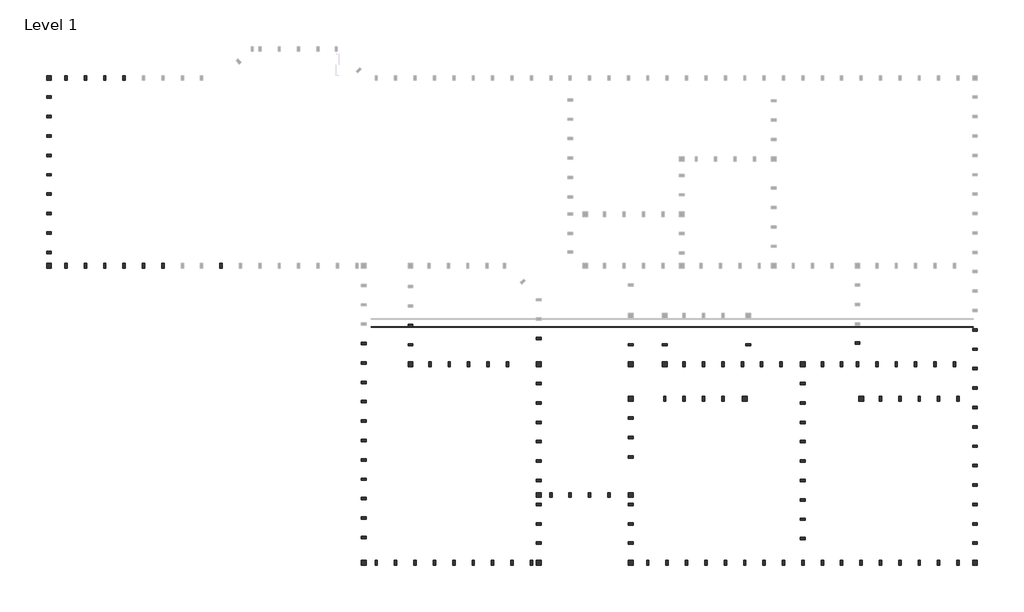
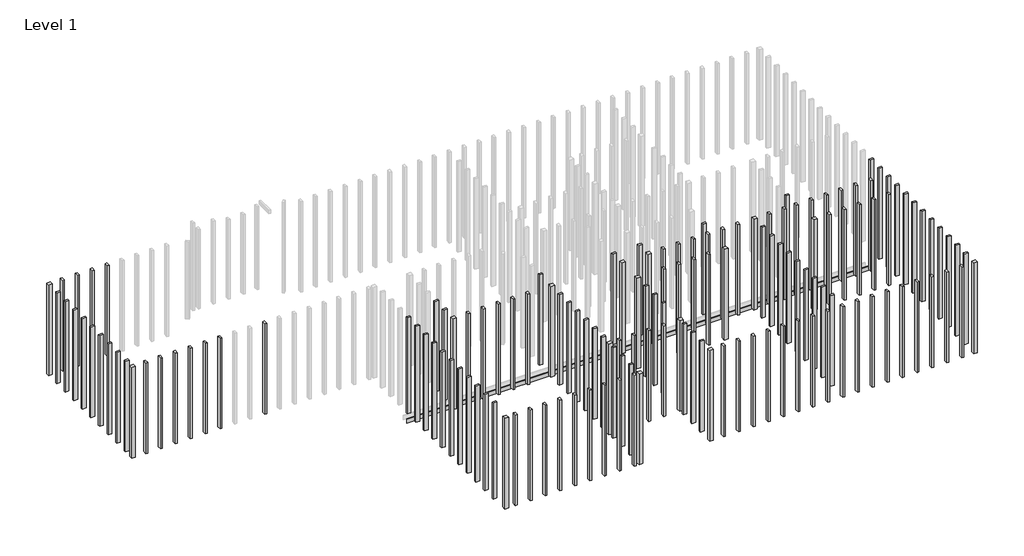
# One storey, part 1 of 2: 148 columns, 1 beam.
"""IFC4 building model written with IfcOpenShell, lengths in millimetres."""

import ifcopenshell
import ifcopenshell.guid

model = None  # the IFC model being written
_history = None  # IfcOwnerHistory: only IFC2X3 demands one
_inside = {}  # id of a spatial element -> (the spatial element, [elements in it])
_under = {}  # id of a project, library or spatial element -> (it, [spatial elements below it])
_declared = {}  # id of a project -> (the project, [libraries it declares])
_typed = {}  # id of a type object -> (the type object, [elements of that type])
_made_of = {}  # id of a material, layer set ... -> (it, [elements and type objects made of it])


def new_model(schema):
    """Start an empty IFC model of exactly this schema.

    Asked for "IFC4X3", IfcOpenShell would pick the latest addendum, in which some entities
    have other attributes; the version numbers below select the first issue.
    IFC2X3 requires an IfcOwnerHistory on every rooted entity: one is made here for all.
    """
    global model, _history
    if schema == "IFC4X3":
        model = ifcopenshell.file(schema_version=(4, 3, 0, 0))
    else:
        model = ifcopenshell.file(schema=schema)
    _inside.clear()
    _under.clear()
    _declared.clear()
    _typed.clear()
    _made_of.clear()
    _history = None
    if model.schema == "IFC2X3":
        org = make("IfcOrganization", Name="unknown")
        user = make(
            "IfcPersonAndOrganization",
            ThePerson=make("IfcPerson", FamilyName="unknown"),
            TheOrganization=org,
        )
        app = make(
            "IfcApplication",
            ApplicationDeveloper=org,
            Version="unknown",
            ApplicationFullName="unknown",
            ApplicationIdentifier="unknown",
        )
        _history = make(
            "IfcOwnerHistory",
            OwningUser=user,
            OwningApplication=app,
            ChangeAction="ADDED",
            CreationDate=0,
        )
    return model


def make(cls, **values):
    """One entity of the class cls with the attributes given. An attribute that is None is left unset."""
    return model.create_entity(
        cls, **{name: value for name, value in values.items() if value is not None}
    )


def rooted(cls, **values):
    """An entity with a GlobalId (a new one), such as an element, a storey or a relation."""
    return make(cls, GlobalId=ifcopenshell.guid.new(), OwnerHistory=_history, **values)


def si_unit(unit_type, name, prefix=None):
    """IfcSIUnit, for example si_unit("LENGTHUNIT", "METRE", prefix="MILLI")."""
    return make("IfcSIUnit", UnitType=unit_type, Prefix=prefix, Name=name)


def assignment(units):
    """IfcUnitAssignment: the units of a project."""
    return None if units is None else make("IfcUnitAssignment", Units=units)


def point(xyz):
    """IfcCartesianPoint."""
    return None if xyz is None else make("IfcCartesianPoint", Coordinates=xyz)


def direction(xyz):
    """IfcDirection."""
    return None if xyz is None else make("IfcDirection", DirectionRatios=xyz)


def frame(location, z_axis=None, x_axis=None):
    """IfcAxis2Placement3D, a coordinate frame: its origin and axes. An axis left out is left unset."""
    return make(
        "IfcAxis2Placement3D",
        Location=point(location),
        Axis=direction(z_axis),
        RefDirection=direction(x_axis),
    )


def origin():
    """The frame at (0, 0, 0) with its axes left unset."""
    return frame((0.0, 0.0, 0.0))


def origin_with_axes():
    """The frame at (0, 0, 0) with the z axis (0, 0, 1) and the x axis (1, 0, 0) written out."""
    return frame((0.0, 0.0, 0.0), z_axis=(0.0, 0.0, 1.0), x_axis=(1.0, 0.0, 0.0))


def place(relative_to, where):
    """IfcLocalPlacement: puts the frame where relative to a parent placement (None: the world)."""
    return make(
        "IfcLocalPlacement", PlacementRelTo=relative_to, RelativePlacement=where
    )


def context(
    kind, dimensions, precision=None, world=None, true_north=None, identifier=None
):
    """IfcGeometricRepresentationContext, for example the 3D "Model" context."""
    return make(
        "IfcGeometricRepresentationContext",
        ContextIdentifier=identifier,
        ContextType=kind,
        CoordinateSpaceDimension=dimensions,
        Precision=precision,
        WorldCoordinateSystem=world,
        TrueNorth=true_north,
    )


def project(units=None, contexts=None):
    """IfcProject with its units and contexts."""
    return rooted(
        "IfcProject",
        Name="project",
        RepresentationContexts=contexts,
        UnitsInContext=assignment(units),
    )


def spatial(cls, under=None, at=None, **own):
    """A site, building, storey or space (cls), placed at a placement, below another one or the project."""
    s = rooted(cls, ObjectPlacement=at, **own)
    if under is not None:
        _under.setdefault(under.id(), (under, []))[1].append(s)
    return s


def polyline(points):
    """IfcPolyline through the points."""
    return make("IfcPolyline", Points=[point(p) for p in points])


def outline(outer, holes=None, kind="AREA"):
    """IfcArbitraryClosedProfileDef: a profile drawn as a closed curve; with holes, ...WithVoids."""
    if holes is None:
        return make("IfcArbitraryClosedProfileDef", ProfileType=kind, OuterCurve=outer)
    return make(
        "IfcArbitraryProfileDefWithVoids",
        ProfileType=kind,
        OuterCurve=outer,
        InnerCurves=holes,
    )


def extrude(swept, where, along, depth):
    """IfcExtrudedAreaSolid: the profile swept, set in the frame where, extruded along a direction by depth."""
    return make(
        "IfcExtrudedAreaSolid",
        SweptArea=swept,
        Position=where,
        ExtrudedDirection=direction(along),
        Depth=depth,
    )


def shape(context_of_items, identifier, shape_type, items):
    """IfcShapeRepresentation: the items that make up one representation, for example the "Body"."""
    return make(
        "IfcShapeRepresentation",
        ContextOfItems=context_of_items,
        RepresentationIdentifier=identifier,
        RepresentationType=shape_type,
        Items=items,
    )


def source(mapping_origin, context_of_items, identifier, shape_type, items):
    """IfcRepresentationMap: a shape defined once, which mapped items show again and again."""
    return make(
        "IfcRepresentationMap",
        MappingOrigin=mapping_origin,
        MappedRepresentation=shape(context_of_items, identifier, shape_type, items),
    )


def transform(
    local_origin,
    x_axis=None,
    y_axis=None,
    z_axis=None,
    scale=None,
    scale2=None,
    scale3=None,
    uniform=True,
):
    """IfcCartesianTransformationOperator3D, or its non-uniform kind. x_axis, y_axis, z_axis: its Axis1, 2, 3."""
    if uniform:
        return make(
            "IfcCartesianTransformationOperator3D",
            Axis1=direction(x_axis),
            Axis2=direction(y_axis),
            LocalOrigin=point(local_origin),
            Scale=scale,
            Axis3=direction(z_axis),
        )
    return make(
        "IfcCartesianTransformationOperator3DnonUniform",
        Axis1=direction(x_axis),
        Axis2=direction(y_axis),
        LocalOrigin=point(local_origin),
        Scale=scale,
        Axis3=direction(z_axis),
        Scale2=scale2,
        Scale3=scale3,
    )


def mapped(mapping_source, mapping_target):
    """IfcMappedItem: shows the shape of a source again, moved by a transform."""
    return make(
        "IfcMappedItem", MappingSource=mapping_source, MappingTarget=mapping_target
    )


def made_of(thing, what):
    """Note that an element or type object is made of a material, layer set ...; save() writes the relation."""
    if what is not None:
        _made_of.setdefault(what.id(), (what, []))[1].append(thing)
    return thing


def element(
    cls,
    number,
    at=None,
    inside=None,
    cuts=None,
    type_object=None,
    material=None,
    context=None,
    identifier="Body",
    shape_type=None,
    held_by="IfcProductDefinitionShape",
    body=None,
    shapes=None,
    **own,
):
    """One element of the class cls, such as IfcWall. Its Tag is "e" and its number.

    at: its placement. inside: the storey or other place that contains it. cuts: it is an
    opening in that element (IfcRelVoidsElement). A single representation is given by context,
    identifier, shape_type and body (its items); several are given by shapes. held_by: the class
    of the entity that holds the representations. save() writes the other relations.
    """
    e = rooted(cls, Tag="e%d" % number, ObjectPlacement=at, **own)
    if body is not None:
        shapes = [shape(context, identifier, shape_type, body)]
    if shapes is not None:
        e.Representation = make(held_by, Representations=shapes)
    if inside is not None:
        _inside.setdefault(inside.id(), (inside, []))[1].append(e)
    if cuts is not None:
        rooted(
            "IfcRelVoidsElement", RelatingBuildingElement=cuts, RelatedOpeningElement=e
        )
    if type_object is not None:
        _typed.setdefault(type_object.id(), (type_object, []))[1].append(e)
    return made_of(e, material)


def aggregate(whole, parts):
    """IfcRelAggregates: a whole, such as a stair, and the parts it consists of."""
    return rooted("IfcRelAggregates", RelatingObject=whole, RelatedObjects=parts)


def save(model, path):
    """Write the relations noted so far, then the file.

    IfcRelAggregates (storeys below a building ...), IfcRelContainedInSpatialStructure (elements
    in a storey), IfcRelDefinesByType, IfcRelAssociatesMaterial and IfcRelDeclares: one each for
    every whole, place, type object, material and project.
    """
    for whole, parts in _under.values():
        aggregate(whole, parts)
    for where, things in _inside.values():
        rooted(
            "IfcRelContainedInSpatialStructure",
            RelatedElements=things,
            RelatingStructure=where,
        )
    for kind, things in _typed.values():
        rooted("IfcRelDefinesByType", RelatedObjects=things, RelatingType=kind)
    for what, things in _made_of.values():
        rooted("IfcRelAssociatesMaterial", RelatedObjects=things, RelatingMaterial=what)
    for by, libraries in _declared.values():
        rooted("IfcRelDeclares", RelatingContext=by, RelatedDefinitions=libraries)
    model.write(path)


def beam_af2566d3(model_context):
    return source(origin(), model_context, "Body", "SweptSolid", [
        extrude(outline(polyline([(6458.3020508, 5.55625), (6458.3020508, -5.55625), (-6159.1479492, -5.55625), (-6159.1479492, 5.55625), (6458.3020508, 5.55625)])), frame((0.0, 0.0, -63.5), z_axis=(0.0, 0.0, 1.0), x_axis=(1.0, 0.0, 0.0)), (0.0, 0.0, 1.0), 127.0),
    ])


def timber_column_65e54e3c(model_context):
    return source(origin(), model_context, "Body", "SweptSolid", [
        extrude(outline(polyline([(25.4, 50.8), (25.4, -50.8), (-25.4, -50.8), (-25.4, 50.8), (25.4, 50.8)])), frame((0.0, 0.0, 50.8), z_axis=(0.0, 0.0, 1.0), x_axis=(1.0, 0.0, 0.0)), (0.0, 0.0, 1.0), 2616.2),
    ])


def timber_column_b7e6a7b9(model_context):
    return source(origin(), model_context, "Body", "SweptSolid", [
        extrude(outline(polyline([(50.8, 50.8), (50.8, -50.8), (-50.8, -50.8), (-50.8, 50.8), (50.8, 50.8)])), frame((0.0, 0.0, 50.8), z_axis=(0.0, 0.0, 1.0), x_axis=(1.0, 0.0, 0.0)), (0.0, 0.0, 1.0), 2616.2),
    ])


def timber_column_c014de30(model_context):
    return source(origin(), model_context, "Body", "SweptSolid", [
        extrude(outline(polyline([(25.4, -50.8), (-25.4, -50.8), (-25.4, 50.8), (25.4, 50.8), (25.4, -50.8)])), frame((0.0, 0.0, 50.8), z_axis=(0.0, 0.0, 1.0), x_axis=(1.0, 0.0, 0.0)), (0.0, 0.0, 1.0), 2616.2),
    ])


def timber_column_7e99ce9a(model_context):
    return source(origin(), model_context, "Body", "SweptSolid", [
        extrude(outline(polyline([(25.4, 50.8), (25.4, -50.8), (-25.4, -50.8), (-25.4, 50.8), (25.4, 50.8)])), origin_with_axes(), (0.0, 0.0, 1.0), 2768.6),
    ])


model = new_model("IFC4")

# Units and contexts
model_context = context("Model", 3, world=origin())
ifc_project = project(units=[si_unit("LENGTHUNIT", "METRE", prefix="MILLI")], contexts=[model_context])

# Site, building, storey
site = spatial("IfcSite", under=ifc_project)
building = spatial("IfcBuilding", under=site)
storey = spatial("IfcBuildingStorey", under=building, Name="Level 1", Elevation=0.0)

# Beam
placement = place(None, origin())
beam_shape = beam_af2566d3(model_context)
element("IfcBeam", 1, ObjectType="Dimension Lumber : BLDG 6241 7/16\" Plywood Spacer", at=placement, inside=storey, context=model_context, shape_type="MappedRepresentation", body=[
    mapped(beam_shape, transform((-4542.0627783, -55.6278386, -510.38125), x_axis=(-1.0, 0.0, 0.0), y_axis=(0.0, -1.0, 0.0), z_axis=(0.0, 0.0, 1.0))),
])

# Columns
timber_column_shape = timber_column_65e54e3c(model_context)
element("IfcColumn", 2, ObjectType="Timber-Column", at=placement, inside=storey, context=model_context, shape_type="MappedRepresentation", body=[
    mapped(timber_column_shape, transform((-17394.814829, 5156.9284114, 0.0), x_axis=(1.0, 0.0, 0.0), y_axis=(0.0, 1.0, 0.0), z_axis=(0.0, 0.0, 1.0))),
])
element("IfcColumn", 3, ObjectType="Timber-Column", at=placement, inside=storey, context=model_context, shape_type="MappedRepresentation", body=[
    mapped(timber_column_shape, transform((-16988.414829, 5156.9284114, 0.0), x_axis=(1.0, 0.0, 0.0), y_axis=(0.0, 1.0, 0.0), z_axis=(0.0, 0.0, 1.0))),
])
element("IfcColumn", 4, ObjectType="Timber-Column", at=placement, inside=storey, context=model_context, shape_type="MappedRepresentation", body=[
    mapped(timber_column_shape, transform((-16582.014829, 5156.9284114, 0.0), x_axis=(1.0, 0.0, 0.0), y_axis=(0.0, 1.0, 0.0), z_axis=(0.0, 0.0, 1.0))),
])
element("IfcColumn", 5, ObjectType="Timber-Column", at=placement, inside=storey, context=model_context, shape_type="MappedRepresentation", body=[
    mapped(timber_column_shape, transform((-16175.614829, 5156.9284114, 0.0), x_axis=(1.0, 0.0, 0.0), y_axis=(0.0, 1.0, 0.0), z_axis=(0.0, 0.0, 1.0))),
])
element("IfcColumn", 6, ObjectType="Timber-Column", at=placement, inside=storey, context=model_context, shape_type="MappedRepresentation", body=[
    mapped(timber_column_shape, transform((1299.585171, -5003.0715886, 0.0), x_axis=(1.0, 0.0, 0.0), y_axis=(0.0, 1.0, 0.0), z_axis=(0.0, 0.0, 1.0))),
])
element("IfcColumn", 7, ObjectType="Timber-Column", at=placement, inside=storey, context=model_context, shape_type="MappedRepresentation", body=[
    mapped(timber_column_shape, transform((893.185171, -5003.0715886, 0.0), x_axis=(1.0, 0.0, 0.0), y_axis=(0.0, 1.0, 0.0), z_axis=(0.0, 0.0, 1.0))),
])
element("IfcColumn", 8, ObjectType="Timber-Column", at=placement, inside=storey, context=model_context, shape_type="MappedRepresentation", body=[
    mapped(timber_column_shape, transform((486.785171, -5003.0715886, 0.0), x_axis=(1.0, 0.0, 0.0), y_axis=(0.0, 1.0, 0.0), z_axis=(0.0, 0.0, 1.0))),
])
element("IfcColumn", 9, ObjectType="Timber-Column", at=placement, inside=storey, context=model_context, shape_type="MappedRepresentation", body=[
    mapped(timber_column_shape, transform((80.385171, -5003.0715886, 0.0), x_axis=(1.0, 0.0, 0.0), y_axis=(0.0, 1.0, 0.0), z_axis=(0.0, 0.0, 1.0))),
])
element("IfcColumn", 10, ObjectType="Timber-Column", at=placement, inside=storey, context=model_context, shape_type="MappedRepresentation", body=[
    mapped(timber_column_shape, transform((-326.014829, -5003.0715886, 0.0), x_axis=(1.0, 0.0, 0.0), y_axis=(0.0, 1.0, 0.0), z_axis=(0.0, 0.0, 1.0))),
])
element("IfcColumn", 11, ObjectType="Timber-Column", at=placement, inside=storey, context=model_context, shape_type="MappedRepresentation", body=[
    mapped(timber_column_shape, transform((-732.414829, -5003.0715886, 0.0), x_axis=(1.0, 0.0, 0.0), y_axis=(0.0, 1.0, 0.0), z_axis=(0.0, 0.0, 1.0))),
])
element("IfcColumn", 12, ObjectType="Timber-Column", at=placement, inside=storey, context=model_context, shape_type="MappedRepresentation", body=[
    mapped(timber_column_shape, transform((-1138.814829, -5003.0715886, 0.0), x_axis=(1.0, 0.0, 0.0), y_axis=(0.0, 1.0, 0.0), z_axis=(0.0, 0.0, 1.0))),
])
element("IfcColumn", 13, ObjectType="Timber-Column", at=placement, inside=storey, context=model_context, shape_type="MappedRepresentation", body=[
    mapped(timber_column_shape, transform((-1545.214829, -5003.0715886, 0.0), x_axis=(1.0, 0.0, 0.0), y_axis=(0.0, 1.0, 0.0), z_axis=(0.0, 0.0, 1.0))),
])
element("IfcColumn", 14, ObjectType="Timber-Column", at=placement, inside=storey, context=model_context, shape_type="MappedRepresentation", body=[
    mapped(timber_column_shape, transform((-1951.614829, -5003.0715886, 0.0), x_axis=(1.0, 0.0, 0.0), y_axis=(0.0, 1.0, 0.0), z_axis=(0.0, 0.0, 1.0))),
])
element("IfcColumn", 15, ObjectType="Timber-Column", at=placement, inside=storey, context=model_context, shape_type="MappedRepresentation", body=[
    mapped(timber_column_shape, transform((-2358.014829, -5003.0715886, 0.0), x_axis=(1.0, 0.0, 0.0), y_axis=(0.0, 1.0, 0.0), z_axis=(0.0, 0.0, 1.0))),
])
element("IfcColumn", 16, ObjectType="Timber-Column", at=placement, inside=storey, context=model_context, shape_type="MappedRepresentation", body=[
    mapped(timber_column_shape, transform((-2764.414829, -5003.0715886, 0.0), x_axis=(1.0, 0.0, 0.0), y_axis=(0.0, 1.0, 0.0), z_axis=(0.0, 0.0, 1.0))),
])
element("IfcColumn", 17, ObjectType="Timber-Column", at=placement, inside=storey, context=model_context, shape_type="MappedRepresentation", body=[
    mapped(timber_column_shape, transform((-3170.814829, -5003.0715886, 0.0), x_axis=(1.0, 0.0, 0.0), y_axis=(0.0, 1.0, 0.0), z_axis=(0.0, 0.0, 1.0))),
])
element("IfcColumn", 18, ObjectType="Timber-Column", at=placement, inside=storey, context=model_context, shape_type="MappedRepresentation", body=[
    mapped(timber_column_shape, transform((-3577.214829, -5003.0715886, 0.0), x_axis=(1.0, 0.0, 0.0), y_axis=(0.0, 1.0, 0.0), z_axis=(0.0, 0.0, 1.0))),
])
element("IfcColumn", 19, ObjectType="Timber-Column", at=placement, inside=storey, context=model_context, shape_type="MappedRepresentation", body=[
    mapped(timber_column_shape, transform((-3983.614829, -5003.0715886, 0.0), x_axis=(1.0, 0.0, 0.0), y_axis=(0.0, 1.0, 0.0), z_axis=(0.0, 0.0, 1.0))),
])
element("IfcColumn", 20, ObjectType="Timber-Column", at=placement, inside=storey, context=model_context, shape_type="MappedRepresentation", body=[
    mapped(timber_column_shape, transform((-4390.014829, -5003.0715886, 0.0), x_axis=(1.0, 0.0, 0.0), y_axis=(0.0, 1.0, 0.0), z_axis=(0.0, 0.0, 1.0))),
])
element("IfcColumn", 21, ObjectType="Timber-Column", at=placement, inside=storey, context=model_context, shape_type="MappedRepresentation", body=[
    mapped(timber_column_shape, transform((-4796.414829, -5003.0715886, 0.0), x_axis=(1.0, 0.0, 0.0), y_axis=(0.0, 1.0, 0.0), z_axis=(0.0, 0.0, 1.0))),
])
element("IfcColumn", 22, ObjectType="Timber-Column", at=placement, inside=storey, context=model_context, shape_type="MappedRepresentation", body=[
    mapped(timber_column_shape, transform((-5202.814829, -5003.0715886, 0.0), x_axis=(1.0, 0.0, 0.0), y_axis=(0.0, 1.0, 0.0), z_axis=(0.0, 0.0, 1.0))),
])
element("IfcColumn", 23, ObjectType="Timber-Column", at=placement, inside=storey, context=model_context, shape_type="MappedRepresentation", body=[
    mapped(timber_column_shape, transform((-6015.614829, -3580.6715886, 0.0), x_axis=(1.0, 0.0, 0.0), y_axis=(0.0, 1.0, 0.0), z_axis=(0.0, 0.0, 1.0))),
])
element("IfcColumn", 24, ObjectType="Timber-Column", at=placement, inside=storey, context=model_context, shape_type="MappedRepresentation", body=[
    mapped(timber_column_shape, transform((-6422.014829, -3580.6715886, 0.0), x_axis=(1.0, 0.0, 0.0), y_axis=(0.0, 1.0, 0.0), z_axis=(0.0, 0.0, 1.0))),
])
element("IfcColumn", 25, ObjectType="Timber-Column", at=placement, inside=storey, context=model_context, shape_type="MappedRepresentation", body=[
    mapped(timber_column_shape, transform((-6828.414829, -3580.6715886, 0.0), x_axis=(1.0, 0.0, 0.0), y_axis=(0.0, 1.0, 0.0), z_axis=(0.0, 0.0, 1.0))),
])
element("IfcColumn", 26, ObjectType="Timber-Column", at=placement, inside=storey, context=model_context, shape_type="MappedRepresentation", body=[
    mapped(timber_column_shape, transform((-7234.814829, -3580.6715886, 0.0), x_axis=(1.0, 0.0, 0.0), y_axis=(0.0, 1.0, 0.0), z_axis=(0.0, 0.0, 1.0))),
])
element("IfcColumn", 27, ObjectType="Timber-Column", at=placement, inside=storey, context=model_context, shape_type="MappedRepresentation", body=[
    mapped(timber_column_shape, transform((-7641.214829, -5003.0715886, 0.0), x_axis=(1.0, 0.0, 0.0), y_axis=(0.0, 1.0, 0.0), z_axis=(0.0, 0.0, 1.0))),
])
element("IfcColumn", 28, ObjectType="Timber-Column", at=placement, inside=storey, context=model_context, shape_type="MappedRepresentation", body=[
    mapped(timber_column_shape, transform((-8047.614829, -5003.0715886, 0.0), x_axis=(1.0, 0.0, 0.0), y_axis=(0.0, 1.0, 0.0), z_axis=(0.0, 0.0, 1.0))),
])
element("IfcColumn", 29, ObjectType="Timber-Column", at=placement, inside=storey, context=model_context, shape_type="MappedRepresentation", body=[
    mapped(timber_column_shape, transform((-8454.014829, -5003.0715886, 0.0), x_axis=(1.0, 0.0, 0.0), y_axis=(0.0, 1.0, 0.0), z_axis=(0.0, 0.0, 1.0))),
])
element("IfcColumn", 30, ObjectType="Timber-Column", at=placement, inside=storey, context=model_context, shape_type="MappedRepresentation", body=[
    mapped(timber_column_shape, transform((-8860.414829, -5003.0715886, 0.0), x_axis=(1.0, 0.0, 0.0), y_axis=(0.0, 1.0, 0.0), z_axis=(0.0, 0.0, 1.0))),
])
element("IfcColumn", 31, ObjectType="Timber-Column", at=placement, inside=storey, context=model_context, shape_type="MappedRepresentation", body=[
    mapped(timber_column_shape, transform((-9266.814829, -5003.0715886, 0.0), x_axis=(1.0, 0.0, 0.0), y_axis=(0.0, 1.0, 0.0), z_axis=(0.0, 0.0, 1.0))),
])
element("IfcColumn", 32, ObjectType="Timber-Column", at=placement, inside=storey, context=model_context, shape_type="MappedRepresentation", body=[
    mapped(timber_column_shape, transform((-9673.214829, -5003.0715886, 0.0), x_axis=(1.0, 0.0, 0.0), y_axis=(0.0, 1.0, 0.0), z_axis=(0.0, 0.0, 1.0))),
])
element("IfcColumn", 33, ObjectType="Timber-Column", at=placement, inside=storey, context=model_context, shape_type="MappedRepresentation", body=[
    mapped(timber_column_shape, transform((-10079.614829, -5003.0715886, 0.0), x_axis=(1.0, 0.0, 0.0), y_axis=(0.0, 1.0, 0.0), z_axis=(0.0, 0.0, 1.0))),
])
element("IfcColumn", 34, ObjectType="Timber-Column", at=placement, inside=storey, context=model_context, shape_type="MappedRepresentation", body=[
    mapped(timber_column_shape, transform((-10486.014829, -5003.0715886, 0.0), x_axis=(1.0, 0.0, 0.0), y_axis=(0.0, 1.0, 0.0), z_axis=(0.0, 0.0, 1.0))),
])
element("IfcColumn", 35, ObjectType="Timber-Column", at=placement, inside=storey, context=model_context, shape_type="MappedRepresentation", body=[
    mapped(timber_column_shape, transform((-10892.414829, -5003.0715886, 0.0), x_axis=(1.0, 0.0, 0.0), y_axis=(0.0, 1.0, 0.0), z_axis=(0.0, 0.0, 1.0))),
])
element("IfcColumn", 36, ObjectType="Timber-Column", at=placement, inside=storey, context=model_context, shape_type="MappedRepresentation", body=[
    mapped(timber_column_shape, transform((-14143.614829, 1226.2784114, 0.0), x_axis=(1.0, 0.0, 0.0), y_axis=(0.0, 1.0, 0.0), z_axis=(0.0, 0.0, 1.0))),
])
element("IfcColumn", 37, ObjectType="Timber-Column", at=placement, inside=storey, context=model_context, shape_type="MappedRepresentation", body=[
    mapped(timber_column_shape, transform((-15362.814829, 1226.2784114, 0.0), x_axis=(1.0, 0.0, 0.0), y_axis=(0.0, 1.0, 0.0), z_axis=(0.0, 0.0, 1.0))),
])
element("IfcColumn", 38, ObjectType="Timber-Column", at=placement, inside=storey, context=model_context, shape_type="MappedRepresentation", body=[
    mapped(timber_column_shape, transform((-15769.214829, 1226.2784114, 0.0), x_axis=(1.0, 0.0, 0.0), y_axis=(0.0, 1.0, 0.0), z_axis=(0.0, 0.0, 1.0))),
])
element("IfcColumn", 39, ObjectType="Timber-Column", at=placement, inside=storey, context=model_context, shape_type="MappedRepresentation", body=[
    mapped(timber_column_shape, transform((-16175.614829, 1226.2784114, 0.0), x_axis=(1.0, 0.0, 0.0), y_axis=(0.0, 1.0, 0.0), z_axis=(0.0, 0.0, 1.0))),
])
element("IfcColumn", 40, ObjectType="Timber-Column", at=placement, inside=storey, context=model_context, shape_type="MappedRepresentation", body=[
    mapped(timber_column_shape, transform((-16582.014829, 1226.2784114, 0.0), x_axis=(1.0, 0.0, 0.0), y_axis=(0.0, 1.0, 0.0), z_axis=(0.0, 0.0, 1.0))),
])
element("IfcColumn", 41, ObjectType="Timber-Column", at=placement, inside=storey, context=model_context, shape_type="MappedRepresentation", body=[
    mapped(timber_column_shape, transform((-16988.414829, 1226.2784114, 0.0), x_axis=(1.0, 0.0, 0.0), y_axis=(0.0, 1.0, 0.0), z_axis=(0.0, 0.0, 1.0))),
])
element("IfcColumn", 42, ObjectType="Timber-Column", at=placement, inside=storey, context=model_context, shape_type="MappedRepresentation", body=[
    mapped(timber_column_shape, transform((-17394.814829, 1226.2784114, 0.0), x_axis=(1.0, 0.0, 0.0), y_axis=(0.0, 1.0, 0.0), z_axis=(0.0, 0.0, 1.0))),
])
element("IfcColumn", 43, ObjectType="Timber-Column", at=placement, inside=storey, context=model_context, shape_type="MappedRepresentation", body=[
    mapped(timber_column_shape, transform((-17750.414829, 4756.8784114, 0.0), x_axis=(0.0, 1.0, 0.0), y_axis=(-1.0, 0.0, 0.0), z_axis=(0.0, 0.0, 1.0))),
])
element("IfcColumn", 44, ObjectType="Timber-Column", at=placement, inside=storey, context=model_context, shape_type="MappedRepresentation", body=[
    mapped(timber_column_shape, transform((-17750.414829, 4350.4784114, 0.0), x_axis=(0.0, 1.0, 0.0), y_axis=(-1.0, 0.0, 0.0), z_axis=(0.0, 0.0, 1.0))),
])
element("IfcColumn", 45, ObjectType="Timber-Column", at=placement, inside=storey, context=model_context, shape_type="MappedRepresentation", body=[
    mapped(timber_column_shape, transform((-17750.414829, 3944.0784114, 0.0), x_axis=(0.0, 1.0, 0.0), y_axis=(-1.0, 0.0, 0.0), z_axis=(0.0, 0.0, 1.0))),
])
element("IfcColumn", 46, ObjectType="Timber-Column", at=placement, inside=storey, context=model_context, shape_type="MappedRepresentation", body=[
    mapped(timber_column_shape, transform((-17750.414829, 3537.6784114, 0.0), x_axis=(0.0, 1.0, 0.0), y_axis=(-1.0, 0.0, 0.0), z_axis=(0.0, 0.0, 1.0))),
])
element("IfcColumn", 47, ObjectType="Timber-Column", at=placement, inside=storey, context=model_context, shape_type="MappedRepresentation", body=[
    mapped(timber_column_shape, transform((-17750.414829, 3131.2784114, 0.0), x_axis=(0.0, 1.0, 0.0), y_axis=(-1.0, 0.0, 0.0), z_axis=(0.0, 0.0, 1.0))),
])
element("IfcColumn", 48, ObjectType="Timber-Column", at=placement, inside=storey, context=model_context, shape_type="MappedRepresentation", body=[
    mapped(timber_column_shape, transform((-17750.414829, 2724.8784114, 0.0), x_axis=(0.0, 1.0, 0.0), y_axis=(-1.0, 0.0, 0.0), z_axis=(0.0, 0.0, 1.0))),
])
element("IfcColumn", 49, ObjectType="Timber-Column", at=placement, inside=storey, context=model_context, shape_type="MappedRepresentation", body=[
    mapped(timber_column_shape, transform((-17750.414829, 2318.4784114, 0.0), x_axis=(0.0, 1.0, 0.0), y_axis=(-1.0, 0.0, 0.0), z_axis=(0.0, 0.0, 1.0))),
])
element("IfcColumn", 50, ObjectType="Timber-Column", at=placement, inside=storey, context=model_context, shape_type="MappedRepresentation", body=[
    mapped(timber_column_shape, transform((-17750.414829, 1912.0784114, 0.0), x_axis=(0.0, 1.0, 0.0), y_axis=(-1.0, 0.0, 0.0), z_axis=(0.0, 0.0, 1.0))),
])
element("IfcColumn", 51, ObjectType="Timber-Column", at=placement, inside=storey, context=model_context, shape_type="MappedRepresentation", body=[
    mapped(timber_column_shape, transform((-17750.414829, 1505.6784114, 0.0), x_axis=(0.0, 1.0, 0.0), y_axis=(-1.0, 0.0, 0.0), z_axis=(0.0, 0.0, 1.0))),
])
element("IfcColumn", 52, ObjectType="Timber-Column", at=placement, inside=storey, context=model_context, shape_type="MappedRepresentation", body=[
    mapped(timber_column_shape, transform((-7488.814829, -301.7056866, 0.0), x_axis=(0.0, 1.0, 0.0), y_axis=(-1.0, 0.0, 0.0), z_axis=(0.0, 0.0, 1.0))),
])
element("IfcColumn", 53, ObjectType="Timber-Column", at=placement, inside=storey, context=model_context, shape_type="MappedRepresentation", body=[
    mapped(timber_column_shape, transform((-9768.464829, -837.4715886, 0.0), x_axis=(1.0, 0.0, 0.0), y_axis=(0.0, 1.0, 0.0), z_axis=(0.0, 0.0, 1.0))),
])
element("IfcColumn", 54, ObjectType="Timber-Column", at=placement, inside=storey, context=model_context, shape_type="MappedRepresentation", body=[
    mapped(timber_column_shape, transform((-9362.064829, -837.4715886, 0.0), x_axis=(1.0, 0.0, 0.0), y_axis=(0.0, 1.0, 0.0), z_axis=(0.0, 0.0, 1.0))),
])
element("IfcColumn", 55, ObjectType="Timber-Column", at=placement, inside=storey, context=model_context, shape_type="MappedRepresentation", body=[
    mapped(timber_column_shape, transform((-8955.664829, -837.4715886, 0.0), x_axis=(1.0, 0.0, 0.0), y_axis=(0.0, 1.0, 0.0), z_axis=(0.0, 0.0, 1.0))),
])
element("IfcColumn", 56, ObjectType="Timber-Column", at=placement, inside=storey, context=model_context, shape_type="MappedRepresentation", body=[
    mapped(timber_column_shape, transform((-8549.264829, -837.4715886, 0.0), x_axis=(1.0, 0.0, 0.0), y_axis=(0.0, 1.0, 0.0), z_axis=(0.0, 0.0, 1.0))),
])
element("IfcColumn", 57, ObjectType="Timber-Column", at=placement, inside=storey, context=model_context, shape_type="MappedRepresentation", body=[
    mapped(timber_column_shape, transform((-8142.864829, -837.4715886, 0.0), x_axis=(1.0, 0.0, 0.0), y_axis=(0.0, 1.0, 0.0), z_axis=(0.0, 0.0, 1.0))),
])
element("IfcColumn", 58, ObjectType="Timber-Column", at=placement, inside=storey, context=model_context, shape_type="MappedRepresentation", body=[
    mapped(timber_column_shape, transform((-7488.814829, -1243.8715886, 0.0), x_axis=(0.0, 1.0, 0.0), y_axis=(-1.0, 0.0, 0.0), z_axis=(0.0, 0.0, 1.0))),
])
element("IfcColumn", 59, ObjectType="Timber-Column", at=placement, inside=storey, context=model_context, shape_type="MappedRepresentation", body=[
    mapped(timber_column_shape, transform((-7488.814829, -1650.2715886, 0.0), x_axis=(0.0, 1.0, 0.0), y_axis=(-1.0, 0.0, 0.0), z_axis=(0.0, 0.0, 1.0))),
])
element("IfcColumn", 60, ObjectType="Timber-Column", at=placement, inside=storey, context=model_context, shape_type="MappedRepresentation", body=[
    mapped(timber_column_shape, transform((-7488.814829, -2056.6715886, 0.0), x_axis=(0.0, 1.0, 0.0), y_axis=(-1.0, 0.0, 0.0), z_axis=(0.0, 0.0, 1.0))),
])
element("IfcColumn", 61, ObjectType="Timber-Column", at=placement, inside=storey, context=model_context, shape_type="MappedRepresentation", body=[
    mapped(timber_column_shape, transform((-7488.814829, -2463.0715886, 0.0), x_axis=(0.0, 1.0, 0.0), y_axis=(-1.0, 0.0, 0.0), z_axis=(0.0, 0.0, 1.0))),
])
element("IfcColumn", 62, ObjectType="Timber-Column", at=placement, inside=storey, context=model_context, shape_type="MappedRepresentation", body=[
    mapped(timber_column_shape, transform((-7488.814829, -2869.4715886, 0.0), x_axis=(0.0, 1.0, 0.0), y_axis=(-1.0, 0.0, 0.0), z_axis=(0.0, 0.0, 1.0))),
])
element("IfcColumn", 63, ObjectType="Timber-Column", at=placement, inside=storey, context=model_context, shape_type="MappedRepresentation", body=[
    mapped(timber_column_shape, transform((-7488.814829, -3275.8715886, 0.0), x_axis=(0.0, 1.0, 0.0), y_axis=(-1.0, 0.0, 0.0), z_axis=(0.0, 0.0, 1.0))),
])
element("IfcColumn", 64, ObjectType="Timber-Column", at=placement, inside=storey, context=model_context, shape_type="MappedRepresentation", body=[
    mapped(timber_column_shape, transform((-10175.1225949, -431.0715886, 0.0), x_axis=(0.0, 1.0, 0.0), y_axis=(-1.0, 0.0, 0.0), z_axis=(0.0, 0.0, 1.0))),
])
element("IfcColumn", 65, ObjectType="Timber-Column", at=placement, inside=storey, context=model_context, shape_type="MappedRepresentation", body=[
    mapped(timber_column_shape, transform((-10175.1225949, -24.6715886, 0.0), x_axis=(0.0, 1.0, 0.0), y_axis=(-1.0, 0.0, 0.0), z_axis=(0.0, 0.0, 1.0))),
])
element("IfcColumn", 66, ObjectType="Timber-Column", at=placement, inside=storey, context=model_context, shape_type="MappedRepresentation", body=[
    mapped(timber_column_shape, transform((-5558.414829, -431.0715886, 0.0), x_axis=(0.0, 1.0, 0.0), y_axis=(-1.0, 0.0, 0.0), z_axis=(0.0, 0.0, 1.0))),
])
element("IfcColumn", 67, ObjectType="Timber-Column", at=placement, inside=storey, context=model_context, shape_type="MappedRepresentation", body=[
    mapped(timber_column_shape, transform((-5558.414829, -1967.7715886, 0.0), x_axis=(0.0, 1.0, 0.0), y_axis=(-1.0, 0.0, 0.0), z_axis=(0.0, 0.0, 1.0))),
])
element("IfcColumn", 68, ObjectType="Timber-Column", at=placement, inside=storey, context=model_context, shape_type="MappedRepresentation", body=[
    mapped(timber_column_shape, transform((-5558.414829, -2374.1715886, 0.0), x_axis=(0.0, 1.0, 0.0), y_axis=(-1.0, 0.0, 0.0), z_axis=(0.0, 0.0, 1.0))),
])
element("IfcColumn", 69, ObjectType="Timber-Column", at=placement, inside=storey, context=model_context, shape_type="MappedRepresentation", body=[
    mapped(timber_column_shape, transform((-5558.414829, -2780.5715886, 0.0), x_axis=(0.0, 1.0, 0.0), y_axis=(-1.0, 0.0, 0.0), z_axis=(0.0, 0.0, 1.0))),
])
element("IfcColumn", 70, ObjectType="Timber-Column", at=placement, inside=storey, context=model_context, shape_type="MappedRepresentation", body=[
    mapped(timber_column_shape, transform((-4847.214829, -1561.3715886, 0.0), x_axis=(-1.0, 0.0, 0.0), y_axis=(0.0, -1.0, 0.0), z_axis=(0.0, 0.0, 1.0))),
])
element("IfcColumn", 71, ObjectType="Timber-Column", at=placement, inside=storey, context=model_context, shape_type="MappedRepresentation", body=[
    mapped(timber_column_shape, transform((-4440.814829, -1561.3715886, 0.0), x_axis=(-1.0, 0.0, 0.0), y_axis=(0.0, -1.0, 0.0), z_axis=(0.0, 0.0, 1.0))),
])
element("IfcColumn", 72, ObjectType="Timber-Column", at=placement, inside=storey, context=model_context, shape_type="MappedRepresentation", body=[
    mapped(timber_column_shape, transform((-4034.414829, -1561.3715886, 0.0), x_axis=(-1.0, 0.0, 0.0), y_axis=(0.0, -1.0, 0.0), z_axis=(0.0, 0.0, 1.0))),
])
element("IfcColumn", 73, ObjectType="Timber-Column", at=placement, inside=storey, context=model_context, shape_type="MappedRepresentation", body=[
    mapped(timber_column_shape, transform((-3628.014829, -1561.3715886, 0.0), x_axis=(-1.0, 0.0, 0.0), y_axis=(0.0, -1.0, 0.0), z_axis=(0.0, 0.0, 1.0))),
])
element("IfcColumn", 74, ObjectType="Timber-Column", at=placement, inside=storey, context=model_context, shape_type="MappedRepresentation", body=[
    mapped(timber_column_shape, transform((-4440.814829, -837.4715886, 0.0), x_axis=(-1.0, 0.0, 0.0), y_axis=(0.0, -1.0, 0.0), z_axis=(0.0, 0.0, 1.0))),
])
element("IfcColumn", 75, ObjectType="Timber-Column", at=placement, inside=storey, context=model_context, shape_type="MappedRepresentation", body=[
    mapped(timber_column_shape, transform((-4034.414829, -837.4715886, 0.0), x_axis=(-1.0, 0.0, 0.0), y_axis=(0.0, -1.0, 0.0), z_axis=(0.0, 0.0, 1.0))),
])
element("IfcColumn", 76, ObjectType="Timber-Column", at=placement, inside=storey, context=model_context, shape_type="MappedRepresentation", body=[
    mapped(timber_column_shape, transform((-3628.014829, -837.4715886, 0.0), x_axis=(-1.0, 0.0, 0.0), y_axis=(0.0, -1.0, 0.0), z_axis=(0.0, 0.0, 1.0))),
])
element("IfcColumn", 77, ObjectType="Timber-Column", at=placement, inside=storey, context=model_context, shape_type="MappedRepresentation", body=[
    mapped(timber_column_shape, transform((-3221.614829, -837.4715886, 0.0), x_axis=(-1.0, 0.0, 0.0), y_axis=(0.0, -1.0, 0.0), z_axis=(0.0, 0.0, 1.0))),
])
element("IfcColumn", 78, ObjectType="Timber-Column", at=placement, inside=storey, context=model_context, shape_type="MappedRepresentation", body=[
    mapped(timber_column_shape, transform((-2815.214829, -837.4715886, 0.0), x_axis=(-1.0, 0.0, 0.0), y_axis=(0.0, -1.0, 0.0), z_axis=(0.0, 0.0, 1.0))),
])
element("IfcColumn", 79, ObjectType="Timber-Column", at=placement, inside=storey, context=model_context, shape_type="MappedRepresentation", body=[
    mapped(timber_column_shape, transform((-2408.814829, -837.4715886, 0.0), x_axis=(-1.0, 0.0, 0.0), y_axis=(0.0, -1.0, 0.0), z_axis=(0.0, 0.0, 1.0))),
])
element("IfcColumn", 80, ObjectType="Timber-Column", at=placement, inside=storey, context=model_context, shape_type="MappedRepresentation", body=[
    mapped(timber_column_shape, transform((-4847.214829, -431.0715886, 0.0), x_axis=(0.0, 1.0, 0.0), y_axis=(-1.0, 0.0, 0.0), z_axis=(0.0, 0.0, 1.0))),
])
element("IfcColumn", 81, ObjectType="Timber-Column", at=placement, inside=storey, context=model_context, shape_type="MappedRepresentation", body=[
    mapped(timber_column_shape, transform((-3094.614829, -431.0715886, 0.0), x_axis=(0.0, 1.0, 0.0), y_axis=(-1.0, 0.0, 0.0), z_axis=(0.0, 0.0, 1.0))),
])
element("IfcColumn", 82, ObjectType="Timber-Column", at=placement, inside=storey, context=model_context, shape_type="MappedRepresentation", body=[
    mapped(timber_column_shape, transform((-1545.214829, -837.4715886, 0.0), x_axis=(-1.0, 0.0, 0.0), y_axis=(0.0, -1.0, 0.0), z_axis=(0.0, 0.0, 1.0))),
])
element("IfcColumn", 83, ObjectType="Timber-Column", at=placement, inside=storey, context=model_context, shape_type="MappedRepresentation", body=[
    mapped(timber_column_shape, transform((-1138.814829, -837.4715886, 0.0), x_axis=(-1.0, 0.0, 0.0), y_axis=(0.0, -1.0, 0.0), z_axis=(0.0, 0.0, 1.0))),
])
element("IfcColumn", 84, ObjectType="Timber-Column", at=placement, inside=storey, context=model_context, shape_type="MappedRepresentation", body=[
    mapped(timber_column_shape, transform((-808.614829, -837.4715886, 0.0), x_axis=(-1.0, 0.0, 0.0), y_axis=(0.0, -1.0, 0.0), z_axis=(0.0, 0.0, 1.0))),
])
element("IfcColumn", 85, ObjectType="Timber-Column", at=placement, inside=storey, context=model_context, shape_type="MappedRepresentation", body=[
    mapped(timber_column_shape, transform((-402.214829, -837.4715886, 0.0), x_axis=(-1.0, 0.0, 0.0), y_axis=(0.0, -1.0, 0.0), z_axis=(0.0, 0.0, 1.0))),
])
element("IfcColumn", 86, ObjectType="Timber-Column", at=placement, inside=storey, context=model_context, shape_type="MappedRepresentation", body=[
    mapped(timber_column_shape, transform((4.185171, -837.4715886, 0.0), x_axis=(-1.0, 0.0, 0.0), y_axis=(0.0, -1.0, 0.0), z_axis=(0.0, 0.0, 1.0))),
])
element("IfcColumn", 87, ObjectType="Timber-Column", at=placement, inside=storey, context=model_context, shape_type="MappedRepresentation", body=[
    mapped(timber_column_shape, transform((410.585171, -837.4715886, 0.0), x_axis=(-1.0, 0.0, 0.0), y_axis=(0.0, -1.0, 0.0), z_axis=(0.0, 0.0, 1.0))),
])
element("IfcColumn", 88, ObjectType="Timber-Column", at=placement, inside=storey, context=model_context, shape_type="MappedRepresentation", body=[
    mapped(timber_column_shape, transform((816.985171, -837.4715886, 0.0), x_axis=(-1.0, 0.0, 0.0), y_axis=(0.0, -1.0, 0.0), z_axis=(0.0, 0.0, 1.0))),
])
element("IfcColumn", 89, ObjectType="Timber-Column", at=placement, inside=storey, context=model_context, shape_type="MappedRepresentation", body=[
    mapped(timber_column_shape, transform((1223.385171, -837.4715886, 0.0), x_axis=(-1.0, 0.0, 0.0), y_axis=(0.0, -1.0, 0.0), z_axis=(0.0, 0.0, 1.0))),
])
element("IfcColumn", 90, ObjectType="Timber-Column", at=placement, inside=storey, context=model_context, shape_type="MappedRepresentation", body=[
    mapped(timber_column_shape, transform((-326.014829, -1561.3715886, 0.0), x_axis=(-1.0, 0.0, 0.0), y_axis=(0.0, -1.0, 0.0), z_axis=(0.0, 0.0, 1.0))),
])
element("IfcColumn", 91, ObjectType="Timber-Column", at=placement, inside=storey, context=model_context, shape_type="MappedRepresentation", body=[
    mapped(timber_column_shape, transform((80.385171, -1561.3715886, 0.0), x_axis=(-1.0, 0.0, 0.0), y_axis=(0.0, -1.0, 0.0), z_axis=(0.0, 0.0, 1.0))),
])
element("IfcColumn", 92, ObjectType="Timber-Column", at=placement, inside=storey, context=model_context, shape_type="MappedRepresentation", body=[
    mapped(timber_column_shape, transform((486.785171, -1561.3715886, 0.0), x_axis=(-1.0, 0.0, 0.0), y_axis=(0.0, -1.0, 0.0), z_axis=(0.0, 0.0, 1.0))),
])
element("IfcColumn", 93, ObjectType="Timber-Column", at=placement, inside=storey, context=model_context, shape_type="MappedRepresentation", body=[
    mapped(timber_column_shape, transform((893.185171, -1561.3715886, 0.0), x_axis=(-1.0, 0.0, 0.0), y_axis=(0.0, -1.0, 0.0), z_axis=(0.0, 0.0, 1.0))),
])
element("IfcColumn", 94, ObjectType="Timber-Column", at=placement, inside=storey, context=model_context, shape_type="MappedRepresentation", body=[
    mapped(timber_column_shape, transform((1299.585171, -1561.3715886, 0.0), x_axis=(-1.0, 0.0, 0.0), y_axis=(0.0, -1.0, 0.0), z_axis=(0.0, 0.0, 1.0))),
])
element("IfcColumn", 95, ObjectType="Timber-Column", at=placement, inside=storey, context=model_context, shape_type="MappedRepresentation", body=[
    mapped(timber_column_shape, transform((-808.614829, -399.3215886, 0.0), x_axis=(0.0, 1.0, 0.0), y_axis=(-1.0, 0.0, 0.0), z_axis=(0.0, 0.0, 1.0))),
])
element("IfcColumn", 96, ObjectType="Timber-Column", at=placement, inside=storey, context=model_context, shape_type="MappedRepresentation", body=[
    mapped(timber_column_shape, transform((-1951.614829, -1243.8715886, 0.0), x_axis=(0.0, 1.0, 0.0), y_axis=(-1.0, 0.0, 0.0), z_axis=(0.0, 0.0, 1.0))),
])
element("IfcColumn", 97, ObjectType="Timber-Column", at=placement, inside=storey, context=model_context, shape_type="MappedRepresentation", body=[
    mapped(timber_column_shape, transform((-1951.614829, -1650.2715886, 0.0), x_axis=(0.0, 1.0, 0.0), y_axis=(-1.0, 0.0, 0.0), z_axis=(0.0, 0.0, 1.0))),
])
element("IfcColumn", 98, ObjectType="Timber-Column", at=placement, inside=storey, context=model_context, shape_type="MappedRepresentation", body=[
    mapped(timber_column_shape, transform((-1951.614829, -2056.6715886, 0.0), x_axis=(0.0, 1.0, 0.0), y_axis=(-1.0, 0.0, 0.0), z_axis=(0.0, 0.0, 1.0))),
])
element("IfcColumn", 99, ObjectType="Timber-Column", at=placement, inside=storey, context=model_context, shape_type="MappedRepresentation", body=[
    mapped(timber_column_shape, transform((-1951.614829, -2463.0715886, 0.0), x_axis=(0.0, 1.0, 0.0), y_axis=(-1.0, 0.0, 0.0), z_axis=(0.0, 0.0, 1.0))),
])
element("IfcColumn", 100, ObjectType="Timber-Column", at=placement, inside=storey, context=model_context, shape_type="MappedRepresentation", body=[
    mapped(timber_column_shape, transform((-1951.614829, -2869.4715886, 0.0), x_axis=(0.0, 1.0, 0.0), y_axis=(-1.0, 0.0, 0.0), z_axis=(0.0, 0.0, 1.0))),
])
element("IfcColumn", 101, ObjectType="Timber-Column", at=placement, inside=storey, context=model_context, shape_type="MappedRepresentation", body=[
    mapped(timber_column_shape, transform((-1951.614829, -3275.8715886, 0.0), x_axis=(0.0, 1.0, 0.0), y_axis=(-1.0, 0.0, 0.0), z_axis=(0.0, 0.0, 1.0))),
])
element("IfcColumn", 102, ObjectType="Timber-Column", at=placement, inside=storey, context=model_context, shape_type="MappedRepresentation", body=[
    mapped(timber_column_shape, transform((-1951.614829, -3682.2715886, 0.0), x_axis=(0.0, 1.0, 0.0), y_axis=(-1.0, 0.0, 0.0), z_axis=(0.0, 0.0, 1.0))),
])
element("IfcColumn", 103, ObjectType="Timber-Column", at=placement, inside=storey, context=model_context, shape_type="MappedRepresentation", body=[
    mapped(timber_column_shape, transform((-1951.614829, -4088.6715886, 0.0), x_axis=(0.0, 1.0, 0.0), y_axis=(-1.0, 0.0, 0.0), z_axis=(0.0, 0.0, 1.0))),
])
element("IfcColumn", 104, ObjectType="Timber-Column", at=placement, inside=storey, context=model_context, shape_type="MappedRepresentation", body=[
    mapped(timber_column_shape, transform((-1951.614829, -4495.0715886, 0.0), x_axis=(0.0, 1.0, 0.0), y_axis=(-1.0, 0.0, 0.0), z_axis=(0.0, 0.0, 1.0))),
])
timber_column_2_shape = timber_column_b7e6a7b9(model_context)
element("IfcColumn", 105, ObjectType="Timber-Column", at=placement, inside=storey, context=model_context, shape_type="MappedRepresentation", body=[
    mapped(timber_column_2_shape, transform((-17750.414829, 5156.9284114, 0.0), x_axis=(1.0, 0.0, 0.0), y_axis=(0.0, 1.0, 0.0), z_axis=(0.0, 0.0, 1.0))),
])
element("IfcColumn", 106, ObjectType="Timber-Column", at=placement, inside=storey, context=model_context, shape_type="MappedRepresentation", body=[
    mapped(timber_column_2_shape, transform((-17750.414829, 1226.2784114, 0.0), x_axis=(1.0, 0.0, 0.0), y_axis=(0.0, 1.0, 0.0), z_axis=(0.0, 0.0, 1.0))),
])
element("IfcColumn", 107, ObjectType="Timber-Column", at=placement, inside=storey, context=model_context, shape_type="MappedRepresentation", body=[
    mapped(timber_column_2_shape, transform((-11152.764829, -5003.0715886, 0.0), x_axis=(1.0, 0.0, 0.0), y_axis=(0.0, 1.0, 0.0), z_axis=(0.0, 0.0, 1.0))),
])
element("IfcColumn", 108, ObjectType="Timber-Column", at=placement, inside=storey, context=model_context, shape_type="MappedRepresentation", body=[
    mapped(timber_column_2_shape, transform((-7488.814829, -5003.0715886, 0.0), x_axis=(1.0, 0.0, 0.0), y_axis=(0.0, 1.0, 0.0), z_axis=(0.0, 0.0, 1.0))),
])
element("IfcColumn", 109, ObjectType="Timber-Column", at=placement, inside=storey, context=model_context, shape_type="MappedRepresentation", body=[
    mapped(timber_column_2_shape, transform((-7488.814829, -3580.6715886, 0.0), x_axis=(1.0, 0.0, 0.0), y_axis=(0.0, 1.0, 0.0), z_axis=(0.0, 0.0, 1.0))),
])
element("IfcColumn", 110, ObjectType="Timber-Column", at=placement, inside=storey, context=model_context, shape_type="MappedRepresentation", body=[
    mapped(timber_column_2_shape, transform((-5558.414829, -3580.6715886, 0.0), x_axis=(1.0, 0.0, 0.0), y_axis=(0.0, 1.0, 0.0), z_axis=(0.0, 0.0, 1.0))),
])
element("IfcColumn", 111, ObjectType="Timber-Column", at=placement, inside=storey, context=model_context, shape_type="MappedRepresentation", body=[
    mapped(timber_column_2_shape, transform((-5558.414829, -5003.0715886, 0.0), x_axis=(1.0, 0.0, 0.0), y_axis=(0.0, 1.0, 0.0), z_axis=(0.0, 0.0, 1.0))),
])
element("IfcColumn", 112, ObjectType="Timber-Column", at=placement, inside=storey, context=model_context, shape_type="MappedRepresentation", body=[
    mapped(timber_column_2_shape, transform((1655.185171, -5003.0715886, 0.0), x_axis=(1.0, 0.0, 0.0), y_axis=(0.0, 1.0, 0.0), z_axis=(0.0, 0.0, 1.0))),
])
element("IfcColumn", 113, ObjectType="Timber-Column", at=placement, inside=storey, context=model_context, shape_type="MappedRepresentation", body=[
    mapped(timber_column_2_shape, transform((-732.414829, -1561.3715886, 0.0), x_axis=(1.0, 0.0, 0.0), y_axis=(0.0, 1.0, 0.0), z_axis=(0.0, 0.0, 1.0))),
])
element("IfcColumn", 114, ObjectType="Timber-Column", at=placement, inside=storey, context=model_context, shape_type="MappedRepresentation", body=[
    mapped(timber_column_2_shape, transform((-1951.614829, -837.4715886, 0.0), x_axis=(1.0, 0.0, 0.0), y_axis=(0.0, 1.0, 0.0), z_axis=(0.0, 0.0, 1.0))),
])
element("IfcColumn", 115, ObjectType="Timber-Column", at=placement, inside=storey, context=model_context, shape_type="MappedRepresentation", body=[
    mapped(timber_column_2_shape, transform((-3170.814829, -1561.3715886, 0.0), x_axis=(1.0, 0.0, 0.0), y_axis=(0.0, 1.0, 0.0), z_axis=(0.0, 0.0, 1.0))),
])
element("IfcColumn", 116, ObjectType="Timber-Column", at=placement, inside=storey, context=model_context, shape_type="MappedRepresentation", body=[
    mapped(timber_column_2_shape, transform((-4847.214829, -837.4715886, 0.0), x_axis=(1.0, 0.0, 0.0), y_axis=(0.0, 1.0, 0.0), z_axis=(0.0, 0.0, 1.0))),
])
element("IfcColumn", 117, ObjectType="Timber-Column", at=placement, inside=storey, context=model_context, shape_type="MappedRepresentation", body=[
    mapped(timber_column_2_shape, transform((-5558.414829, -837.4715886, 0.0), x_axis=(1.0, 0.0, 0.0), y_axis=(0.0, 1.0, 0.0), z_axis=(0.0, 0.0, 1.0))),
])
element("IfcColumn", 118, ObjectType="Timber-Column", at=placement, inside=storey, context=model_context, shape_type="MappedRepresentation", body=[
    mapped(timber_column_2_shape, transform((-5558.414829, -1561.3715886, 0.0), x_axis=(1.0, 0.0, 0.0), y_axis=(0.0, 1.0, 0.0), z_axis=(0.0, 0.0, 1.0))),
])
element("IfcColumn", 119, ObjectType="Timber-Column", at=placement, inside=storey, context=model_context, shape_type="MappedRepresentation", body=[
    mapped(timber_column_2_shape, transform((-7488.814829, -837.4715886, 0.0), x_axis=(1.0, 0.0, 0.0), y_axis=(0.0, 1.0, 0.0), z_axis=(0.0, 0.0, 1.0))),
])
element("IfcColumn", 120, ObjectType="Timber-Column", at=placement, inside=storey, context=model_context, shape_type="MappedRepresentation", body=[
    mapped(timber_column_2_shape, transform((-10174.864829, -837.4715886, 0.0), x_axis=(1.0, 0.0, 0.0), y_axis=(0.0, 1.0, 0.0), z_axis=(0.0, 0.0, 1.0))),
])
timber_column_3_shape = timber_column_c014de30(model_context)
element("IfcColumn", 121, ObjectType="Timber-Column", at=placement, inside=storey, context=model_context, shape_type="MappedRepresentation", body=[
    mapped(timber_column_3_shape, transform((1655.185171, -119.9215886, 0.0), x_axis=(0.0, 1.0, 0.0), y_axis=(-1.0, 0.0, 0.0), z_axis=(0.0, 0.0, 1.0))),
])
element("IfcColumn", 122, ObjectType="Timber-Column", at=placement, inside=storey, context=model_context, shape_type="MappedRepresentation", body=[
    mapped(timber_column_3_shape, transform((1655.185171, -526.3215886, 0.0), x_axis=(0.0, 1.0, 0.0), y_axis=(-1.0, 0.0, 0.0), z_axis=(0.0, 0.0, 1.0))),
])
element("IfcColumn", 123, ObjectType="Timber-Column", at=placement, inside=storey, context=model_context, shape_type="MappedRepresentation", body=[
    mapped(timber_column_3_shape, transform((1655.185171, -932.7215886, 0.0), x_axis=(0.0, 1.0, 0.0), y_axis=(-1.0, 0.0, 0.0), z_axis=(0.0, 0.0, 1.0))),
])
element("IfcColumn", 124, ObjectType="Timber-Column", at=placement, inside=storey, context=model_context, shape_type="MappedRepresentation", body=[
    mapped(timber_column_3_shape, transform((1655.185171, -1339.1215886, 0.0), x_axis=(0.0, 1.0, 0.0), y_axis=(-1.0, 0.0, 0.0), z_axis=(0.0, 0.0, 1.0))),
])
element("IfcColumn", 125, ObjectType="Timber-Column", at=placement, inside=storey, context=model_context, shape_type="MappedRepresentation", body=[
    mapped(timber_column_3_shape, transform((1655.185171, -1745.5215886, 0.0), x_axis=(0.0, 1.0, 0.0), y_axis=(-1.0, 0.0, 0.0), z_axis=(0.0, 0.0, 1.0))),
])
element("IfcColumn", 126, ObjectType="Timber-Column", at=placement, inside=storey, context=model_context, shape_type="MappedRepresentation", body=[
    mapped(timber_column_3_shape, transform((1655.185171, -2151.9215886, 0.0), x_axis=(0.0, 1.0, 0.0), y_axis=(-1.0, 0.0, 0.0), z_axis=(0.0, 0.0, 1.0))),
])
element("IfcColumn", 127, ObjectType="Timber-Column", at=placement, inside=storey, context=model_context, shape_type="MappedRepresentation", body=[
    mapped(timber_column_3_shape, transform((1655.185171, -2558.3215886, 0.0), x_axis=(0.0, 1.0, 0.0), y_axis=(-1.0, 0.0, 0.0), z_axis=(0.0, 0.0, 1.0))),
])
element("IfcColumn", 128, ObjectType="Timber-Column", at=placement, inside=storey, context=model_context, shape_type="MappedRepresentation", body=[
    mapped(timber_column_3_shape, transform((1655.185171, -2964.7215886, 0.0), x_axis=(0.0, 1.0, 0.0), y_axis=(-1.0, 0.0, 0.0), z_axis=(0.0, 0.0, 1.0))),
])
element("IfcColumn", 129, ObjectType="Timber-Column", at=placement, inside=storey, context=model_context, shape_type="MappedRepresentation", body=[
    mapped(timber_column_3_shape, transform((1655.185171, -3371.1215886, 0.0), x_axis=(0.0, 1.0, 0.0), y_axis=(-1.0, 0.0, 0.0), z_axis=(0.0, 0.0, 1.0))),
])
element("IfcColumn", 130, ObjectType="Timber-Column", at=placement, inside=storey, context=model_context, shape_type="MappedRepresentation", body=[
    mapped(timber_column_3_shape, transform((1655.185171, -3777.5215886, 0.0), x_axis=(0.0, 1.0, 0.0), y_axis=(-1.0, 0.0, 0.0), z_axis=(0.0, 0.0, 1.0))),
])
element("IfcColumn", 131, ObjectType="Timber-Column", at=placement, inside=storey, context=model_context, shape_type="MappedRepresentation", body=[
    mapped(timber_column_3_shape, transform((1655.185171, -4183.9215886, 0.0), x_axis=(0.0, 1.0, 0.0), y_axis=(-1.0, 0.0, 0.0), z_axis=(0.0, 0.0, 1.0))),
])
element("IfcColumn", 132, ObjectType="Timber-Column", at=placement, inside=storey, context=model_context, shape_type="MappedRepresentation", body=[
    mapped(timber_column_3_shape, transform((1655.185171, -4590.3215886, 0.0), x_axis=(0.0, 1.0, 0.0), y_axis=(-1.0, 0.0, 0.0), z_axis=(0.0, 0.0, 1.0))),
])
element("IfcColumn", 133, ObjectType="Timber-Column", at=placement, inside=storey, context=model_context, shape_type="MappedRepresentation", body=[
    mapped(timber_column_3_shape, transform((-5558.414829, -4590.3215886, 0.0), x_axis=(0.0, 1.0, 0.0), y_axis=(-1.0, 0.0, 0.0), z_axis=(0.0, 0.0, 1.0))),
])
element("IfcColumn", 134, ObjectType="Timber-Column", at=placement, inside=storey, context=model_context, shape_type="MappedRepresentation", body=[
    mapped(timber_column_3_shape, transform((-5558.414829, -4183.9215886, 0.0), x_axis=(0.0, 1.0, 0.0), y_axis=(-1.0, 0.0, 0.0), z_axis=(0.0, 0.0, 1.0))),
])
element("IfcColumn", 135, ObjectType="Timber-Column", at=placement, inside=storey, context=model_context, shape_type="MappedRepresentation", body=[
    mapped(timber_column_3_shape, transform((-5558.414829, -3777.5215886, 0.0), x_axis=(0.0, 1.0, 0.0), y_axis=(-1.0, 0.0, 0.0), z_axis=(0.0, 0.0, 1.0))),
])
element("IfcColumn", 136, ObjectType="Timber-Column", at=placement, inside=storey, context=model_context, shape_type="MappedRepresentation", body=[
    mapped(timber_column_3_shape, transform((-7488.814829, -4590.3215886, 0.0), x_axis=(0.0, 1.0, 0.0), y_axis=(-1.0, 0.0, 0.0), z_axis=(0.0, 0.0, 1.0))),
])
element("IfcColumn", 137, ObjectType="Timber-Column", at=placement, inside=storey, context=model_context, shape_type="MappedRepresentation", body=[
    mapped(timber_column_3_shape, transform((-7488.814829, -4183.9215886, 0.0), x_axis=(0.0, 1.0, 0.0), y_axis=(-1.0, 0.0, 0.0), z_axis=(0.0, 0.0, 1.0))),
])
element("IfcColumn", 138, ObjectType="Timber-Column", at=placement, inside=storey, context=model_context, shape_type="MappedRepresentation", body=[
    mapped(timber_column_3_shape, transform((-7488.814829, -3777.5215886, 0.0), x_axis=(0.0, 1.0, 0.0), y_axis=(-1.0, 0.0, 0.0), z_axis=(0.0, 0.0, 1.0))),
])
timber_column_4_shape = timber_column_7e99ce9a(model_context)
element("IfcColumn", 139, ObjectType="Timber-Column", at=placement, inside=storey, context=model_context, shape_type="MappedRepresentation", body=[
    mapped(timber_column_4_shape, transform((-11152.764829, -405.6715886, 0.0), x_axis=(0.0, 1.0, 0.0), y_axis=(-1.0, 0.0, 0.0), z_axis=(0.0, 0.0, 1.0))),
])
element("IfcColumn", 140, ObjectType="Timber-Column", at=placement, inside=storey, context=model_context, shape_type="MappedRepresentation", body=[
    mapped(timber_column_4_shape, transform((-11152.764829, -812.0715886, 0.0), x_axis=(0.0, 1.0, 0.0), y_axis=(-1.0, 0.0, 0.0), z_axis=(0.0, 0.0, 1.0))),
])
element("IfcColumn", 141, ObjectType="Timber-Column", at=placement, inside=storey, context=model_context, shape_type="MappedRepresentation", body=[
    mapped(timber_column_4_shape, transform((-11152.764829, -1218.4715886, 0.0), x_axis=(0.0, 1.0, 0.0), y_axis=(-1.0, 0.0, 0.0), z_axis=(0.0, 0.0, 1.0))),
])
element("IfcColumn", 142, ObjectType="Timber-Column", at=placement, inside=storey, context=model_context, shape_type="MappedRepresentation", body=[
    mapped(timber_column_4_shape, transform((-11152.764829, -1624.8715886, 0.0), x_axis=(0.0, 1.0, 0.0), y_axis=(-1.0, 0.0, 0.0), z_axis=(0.0, 0.0, 1.0))),
])
element("IfcColumn", 143, ObjectType="Timber-Column", at=placement, inside=storey, context=model_context, shape_type="MappedRepresentation", body=[
    mapped(timber_column_4_shape, transform((-11152.764829, -2031.2715886, 0.0), x_axis=(0.0, 1.0, 0.0), y_axis=(-1.0, 0.0, 0.0), z_axis=(0.0, 0.0, 1.0))),
])
element("IfcColumn", 144, ObjectType="Timber-Column", at=placement, inside=storey, context=model_context, shape_type="MappedRepresentation", body=[
    mapped(timber_column_4_shape, transform((-11152.764829, -2437.6715886, 0.0), x_axis=(0.0, 1.0, 0.0), y_axis=(-1.0, 0.0, 0.0), z_axis=(0.0, 0.0, 1.0))),
])
element("IfcColumn", 145, ObjectType="Timber-Column", at=placement, inside=storey, context=model_context, shape_type="MappedRepresentation", body=[
    mapped(timber_column_4_shape, transform((-11152.764829, -2844.0715886, 0.0), x_axis=(0.0, 1.0, 0.0), y_axis=(-1.0, 0.0, 0.0), z_axis=(0.0, 0.0, 1.0))),
])
element("IfcColumn", 146, ObjectType="Timber-Column", at=placement, inside=storey, context=model_context, shape_type="MappedRepresentation", body=[
    mapped(timber_column_4_shape, transform((-11152.764829, -3250.4715886, 0.0), x_axis=(0.0, 1.0, 0.0), y_axis=(-1.0, 0.0, 0.0), z_axis=(0.0, 0.0, 1.0))),
])
element("IfcColumn", 147, ObjectType="Timber-Column", at=placement, inside=storey, context=model_context, shape_type="MappedRepresentation", body=[
    mapped(timber_column_4_shape, transform((-11152.764829, -3656.8715886, 0.0), x_axis=(0.0, 1.0, 0.0), y_axis=(-1.0, 0.0, 0.0), z_axis=(0.0, 0.0, 1.0))),
])
element("IfcColumn", 148, ObjectType="Timber-Column", at=placement, inside=storey, context=model_context, shape_type="MappedRepresentation", body=[
    mapped(timber_column_4_shape, transform((-11152.764829, -4063.2715886, 0.0), x_axis=(0.0, 1.0, 0.0), y_axis=(-1.0, 0.0, 0.0), z_axis=(0.0, 0.0, 1.0))),
])
element("IfcColumn", 149, ObjectType="Timber-Column", at=placement, inside=storey, context=model_context, shape_type="MappedRepresentation", body=[
    mapped(timber_column_4_shape, transform((-11152.764829, -4469.6715886, 0.0), x_axis=(0.0, 1.0, 0.0), y_axis=(-1.0, 0.0, 0.0), z_axis=(0.0, 0.0, 1.0))),
])

save(model, "model.ifc")

# Revit data of these elements
# Type "Dimension Lumber : BLDG 6241 7/16\" Plywood Spacer"
#   Assembly Code = "B10"
#   A = 0.273472 SF
#   Length [instance default] = 5' - 0"
#   b = 0' - 0 7/16"
#   d = 0' - 5"
#   Structural Material [instance default] = Softwood, Lumber
# Type "Timber-Column : BLDG 6241 Wall Struds 2\"x4\""
#   Assembly Code = "B10"
#   A = 0.140625 SF
#   b = 0' - 2"
#   d = 0' - 4"
#   Structural Material [instance default] = Softwood, Lumber
# Type "Timber-Column : BLDG 6241 Wall Struds 4\"x4\""
#   Assembly Code = "B10"
#   A = 0.140625 SF
#   b = 0' - 4"
#   d = 0' - 4"
#   Structural Material [instance default] = Softwood, Lumber
# Element 1 (IfcBeam, "Dimension Lumber : BLDG 6241 7/16\" Plywood Spacer")
#   Comments = ""
#   Structural Material = Plywood, Sheathing
#   Phase Created = New Construction
#   Materials on its faces: "Plywood, Sheathing"
# Elements 2, 3, 4, 5, 6, 7, 8, 9, 10, 11, 12, 13, 14, 15, 16, 17, 18, 19, 20, 21, 22, 23, 24, 25, 26, 27, 28, 29, 30, 31, 32, 33, 34, 35, 36, 37, 38, 39, 40, 41, 42, 43, 44, 45, 46, 47, 48, 49, 50, 51, 52, 53, 54, 55, 56, 57, 58, 59, 60, 61, 62, 63, 64, 65, 66, 67, 68, 69, 70, 71, 72, 73, 74, 75, 76, 77, 78, 79, 80, 81, 82, 83, 84, 85, 86, 87, 88, 89, 90, 91, 92, 93, 94, 95, 96, 97, 98, 99, 100, 101, 102, 103, 104, 121, 122, 123, 124, 125, 126, 127, 128, 129, 130, 131, 132, 133, 134, 135, 136, 137, 138, 139, 140, 141, 142, 143, 144, 145, 146, 147, 148, 149 (IfcColumn, "Timber-Column : BLDG 6241 Wall Struds 2\"x4\"")
#   Comments = ""
#   Structural Material = Softwood, Lumber
#   Phase Created = New Construction
#   Materials on its faces: "Softwood, Lumber"
